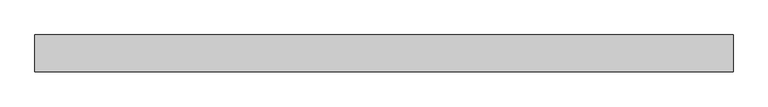
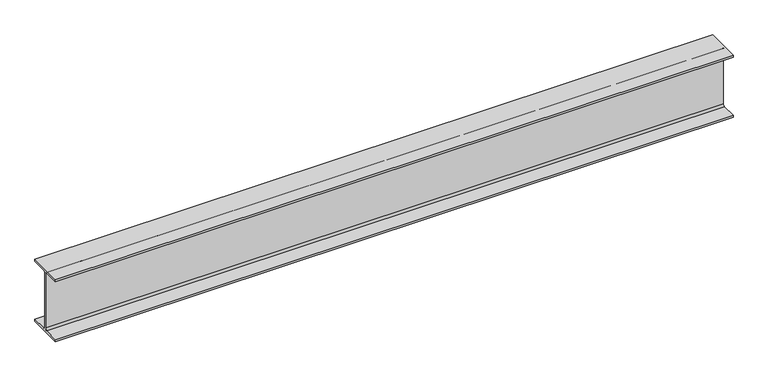
"""IFC4 building model written with IfcOpenShell, lengths in millimetres: beam geometry, Old_Steel Beam_H-KSD3502 : H_SB_ASB_H-200×200x8x12."""

from ifc_helpers import new_model, si_unit, point, frame, frame_2d, origin, place, context, project, spatial, polyline, circle_curve, trimmed, segment, composite_curve, outline, extrude, source, transform, mapped, element, save


def beam_113fc680(model_context):
    return source(origin(), model_context, "Body", "SweptSolid", [
        extrude(outline(composite_curve([segment(polyline([(82.5, -141.5), (82.5, -151.7), (-82.5, -151.7), (-82.5, -141.5), (-11.9, -141.5)]), True, "CONTINUOUS"), segment(trimmed(circle_curve(frame_2d((-11.9, -132.6)), 8.9), [point((-11.9, -141.5))], [point((-3.0, -132.6))], True, "CARTESIAN"), True, "CONTINUOUS"), segment(polyline([(-3.0, -132.6), (-3.0, 132.6)]), True, "CONTINUOUS"), segment(trimmed(circle_curve(frame_2d((-11.9, 132.6)), 8.9), [point((-3.0, 132.6))], [point((-11.9, 141.5))], True, "CARTESIAN"), True, "CONTINUOUS"), segment(polyline([(-11.9, 141.5), (-82.5, 141.5), (-82.5, 151.7), (82.5, 151.7), (82.5, 141.5), (11.9, 141.5)]), True, "CONTINUOUS"), segment(trimmed(circle_curve(frame_2d((11.9, 132.6)), 8.9), [point((11.9, 141.5))], [point((3.0, 132.6))], True, "CARTESIAN"), True, "CONTINUOUS"), segment(polyline([(3.0, 132.6), (3.0, -132.6)]), True, "CONTINUOUS"), segment(trimmed(circle_curve(frame_2d((11.9, -132.6)), 8.9), [point((3.0, -132.6))], [point((11.9, -141.5))], True, "CARTESIAN"), True, "CONTINUOUS"), segment(polyline([(11.9, -141.5), (82.5, -141.5)]), True, "CONTINUOUS")], self_intersect=False)), frame((-1415.6048683, 0.0, 0.0), z_axis=(1.0, 0.0, 0.0), x_axis=(0.0, 1.0, 0.0)), (0.0, 0.0, 1.0), 3137.3489485),
    ])


if __name__ == "__main__":
    model = new_model("IFC4")
    model_context = context("Model", 3, world=origin())
    ifc_project = project(units=[si_unit("LENGTHUNIT", "METRE", prefix="MILLI")], contexts=[model_context])
    site = spatial("IfcSite", under=ifc_project)
    building = spatial("IfcBuilding", under=site)
    placement = place(None, origin())
    beam_shape = beam_113fc680(model_context)
    element("IfcBeam", 1, ObjectType="Old_Steel Beam_H-KSD3502 : H_SB_ASB_H-200×200x8x12", at=placement, inside=building, context=model_context, shape_type="MappedRepresentation", body=[
        mapped(beam_shape, transform((0.0, 0.0, 0.0), x_axis=(1.0, 0.0, 0.0), y_axis=(0.0, 1.0, 0.0), z_axis=(0.0, 0.0, 1.0))),
    ])
    save(model, "model.ifc")

# Revit data of these elements
# Type "Old_Steel Beam_H-KSD3502 : H_SB_ASB_H-200×200x8x12"
#   Width = 20.0 cm
#   Web Thickness = 0.8 cm
#   Web Fillet = 1.3 cm
#   Warping Constant = 141376.0 cm⁶
#   Torsional Moment of Inertia = 26.2485 cm⁴
#   Torsional Modulus = 1.0 cm³
#   Section Area = 63.53 cm²
#   Plastic Modulus weak axis = 244.0 cm³
#   Plastic Modulus strong axis = 525.0 cm³
#   Perimeter = 1.16 m²/m
#   Nominal Weight = 49.90 kgf/m
#   Moment of Inertia weak axis = 1600.00 cm⁴
#   Moment of Inertia strong axis = 4720.00 cm⁴
#   Height = 20.0 cm
#   Flange Thickness = 1.2 cm
#   Elastic Modulus weak axis = 160.0 cm³
#   Elastic Modulus strong axis = 472.0 cm³
#   Centroid Vertical = 10.0 cm
#   Centroid Horizontal = 10.0 cm
#   Length [instance default] = 1.5240 m
#   Structural Material [instance default] = Steel, 45-345
#   Assembly Code = ""
# Element 1 (IfcBeam, "Old_Steel Beam_H-KSD3502 : H_SB_ASB_H-200×200x8x12")
#   Structural Material = none
# Materials
#   "Steel, 45-345": class "Metal", colour RGB 189 187 185, transparency 0, Description = "Steel 345 MPa", Cost = 0
